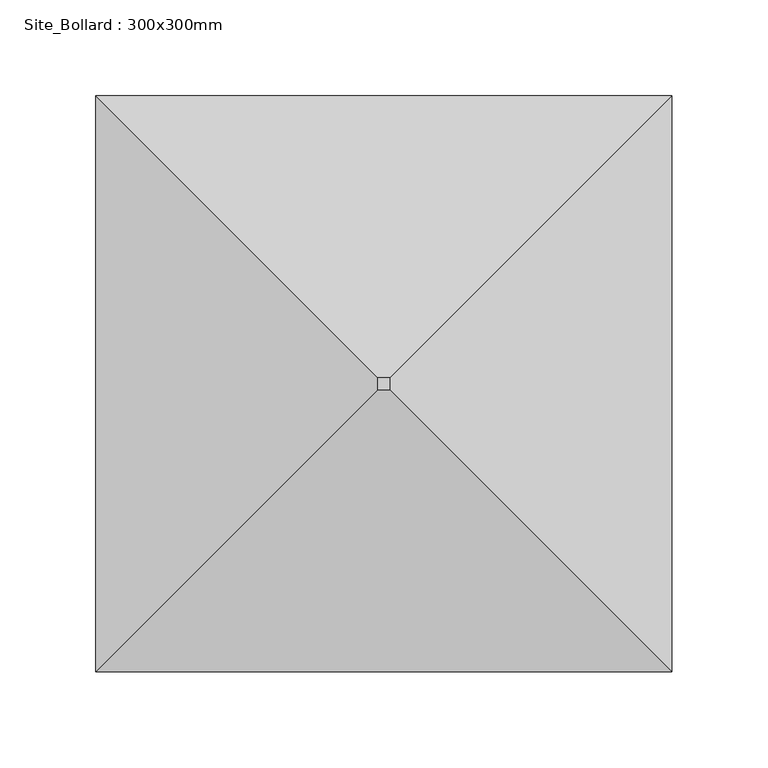
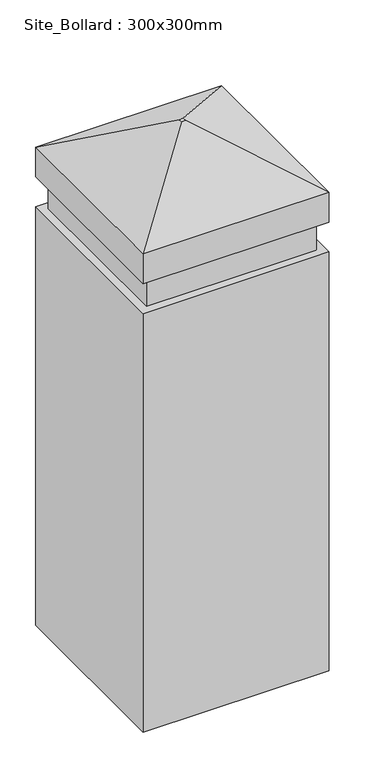
"""IFC4 building model written with IfcOpenShell, lengths in millimetres: geographic element geometry, Site_Bollard : 300x300mm."""

import ifcopenshell
import ifcopenshell.guid

model = None  # the IFC model being written
_history = None  # IfcOwnerHistory: only IFC2X3 demands one
_inside = {}  # id of a spatial element -> (the spatial element, [elements in it])
_under = {}  # id of a project, library or spatial element -> (it, [spatial elements below it])
_declared = {}  # id of a project -> (the project, [libraries it declares])
_typed = {}  # id of a type object -> (the type object, [elements of that type])
_made_of = {}  # id of a material, layer set ... -> (it, [elements and type objects made of it])


def new_model(schema):
    """Start an empty IFC model of exactly this schema.

    Asked for "IFC4X3", IfcOpenShell would pick the latest addendum, in which some entities
    have other attributes; the version numbers below select the first issue.
    IFC2X3 requires an IfcOwnerHistory on every rooted entity: one is made here for all.
    """
    global model, _history
    if schema == "IFC4X3":
        model = ifcopenshell.file(schema_version=(4, 3, 0, 0))
    else:
        model = ifcopenshell.file(schema=schema)
    _inside.clear()
    _under.clear()
    _declared.clear()
    _typed.clear()
    _made_of.clear()
    _history = None
    if model.schema == "IFC2X3":
        org = make("IfcOrganization", Name="unknown")
        user = make(
            "IfcPersonAndOrganization",
            ThePerson=make("IfcPerson", FamilyName="unknown"),
            TheOrganization=org,
        )
        app = make(
            "IfcApplication",
            ApplicationDeveloper=org,
            Version="unknown",
            ApplicationFullName="unknown",
            ApplicationIdentifier="unknown",
        )
        _history = make(
            "IfcOwnerHistory",
            OwningUser=user,
            OwningApplication=app,
            ChangeAction="ADDED",
            CreationDate=0,
        )
    return model


def make(cls, **values):
    """One entity of the class cls with the attributes given. An attribute that is None is left unset."""
    return model.create_entity(
        cls, **{name: value for name, value in values.items() if value is not None}
    )


def rooted(cls, **values):
    """An entity with a GlobalId (a new one), such as an element, a storey or a relation."""
    return make(cls, GlobalId=ifcopenshell.guid.new(), OwnerHistory=_history, **values)


def si_unit(unit_type, name, prefix=None):
    """IfcSIUnit, for example si_unit("LENGTHUNIT", "METRE", prefix="MILLI")."""
    return make("IfcSIUnit", UnitType=unit_type, Prefix=prefix, Name=name)


def assignment(units):
    """IfcUnitAssignment: the units of a project."""
    return None if units is None else make("IfcUnitAssignment", Units=units)


def point(xyz):
    """IfcCartesianPoint."""
    return None if xyz is None else make("IfcCartesianPoint", Coordinates=xyz)


def direction(xyz):
    """IfcDirection."""
    return None if xyz is None else make("IfcDirection", DirectionRatios=xyz)


def frame(location, z_axis=None, x_axis=None):
    """IfcAxis2Placement3D, a coordinate frame: its origin and axes. An axis left out is left unset."""
    return make(
        "IfcAxis2Placement3D",
        Location=point(location),
        Axis=direction(z_axis),
        RefDirection=direction(x_axis),
    )


def origin():
    """The frame at (0, 0, 0) with its axes left unset."""
    return frame((0.0, 0.0, 0.0))


def origin_with_axes():
    """The frame at (0, 0, 0) with the z axis (0, 0, 1) and the x axis (1, 0, 0) written out."""
    return frame((0.0, 0.0, 0.0), z_axis=(0.0, 0.0, 1.0), x_axis=(1.0, 0.0, 0.0))


def place(relative_to, where):
    """IfcLocalPlacement: puts the frame where relative to a parent placement (None: the world)."""
    return make(
        "IfcLocalPlacement", PlacementRelTo=relative_to, RelativePlacement=where
    )


def context(
    kind, dimensions, precision=None, world=None, true_north=None, identifier=None
):
    """IfcGeometricRepresentationContext, for example the 3D "Model" context."""
    return make(
        "IfcGeometricRepresentationContext",
        ContextIdentifier=identifier,
        ContextType=kind,
        CoordinateSpaceDimension=dimensions,
        Precision=precision,
        WorldCoordinateSystem=world,
        TrueNorth=true_north,
    )


def project(units=None, contexts=None):
    """IfcProject with its units and contexts."""
    return rooted(
        "IfcProject",
        Name="project",
        RepresentationContexts=contexts,
        UnitsInContext=assignment(units),
    )


def spatial(cls, under=None, at=None, **own):
    """A site, building, storey or space (cls), placed at a placement, below another one or the project."""
    s = rooted(cls, ObjectPlacement=at, **own)
    if under is not None:
        _under.setdefault(under.id(), (under, []))[1].append(s)
    return s


def polyline(points):
    """IfcPolyline through the points."""
    return make("IfcPolyline", Points=[point(p) for p in points])


def outline(outer, holes=None, kind="AREA"):
    """IfcArbitraryClosedProfileDef: a profile drawn as a closed curve; with holes, ...WithVoids."""
    if holes is None:
        return make("IfcArbitraryClosedProfileDef", ProfileType=kind, OuterCurve=outer)
    return make(
        "IfcArbitraryProfileDefWithVoids",
        ProfileType=kind,
        OuterCurve=outer,
        InnerCurves=holes,
    )


def extrude(swept, where, along, depth):
    """IfcExtrudedAreaSolid: the profile swept, set in the frame where, extruded along a direction by depth."""
    return make(
        "IfcExtrudedAreaSolid",
        SweptArea=swept,
        Position=where,
        ExtrudedDirection=direction(along),
        Depth=depth,
    )


def faces_of(points, faces, orient=None, outer=None):
    """IfcFace entities. A face is a list of loops; a loop is a list of indices into points, from 0.

    orient and outer hold one flag for each loop. By default every Orientation is true, the
    first loop of a face is its IfcFaceOuterBound and the others are IfcFaceBound.
    """
    made = []
    for i, loops in enumerate(faces):
        bounds = []
        for j, loop in enumerate(loops):
            is_outer = j == 0 if outer is None else outer[i][j]
            bounds.append(
                make(
                    "IfcFaceOuterBound" if is_outer else "IfcFaceBound",
                    Bound=make("IfcPolyLoop", Polygon=[points[k] for k in loop]),
                    Orientation=True if orient is None else orient[i][j],
                )
            )
        made.append(make("IfcFace", Bounds=bounds))
    return made


def faceted_brep(points, faces, orient=None, outer=None, voids=None):
    """IfcFacetedBrep: a solid bounded by flat faces; with voids (closed shells), ...WithVoids."""
    shared = [point(p) for p in points]
    hull = make("IfcClosedShell", CfsFaces=faces_of(shared, faces, orient, outer))
    if voids is None:
        return make("IfcFacetedBrep", Outer=hull)
    return make(
        "IfcFacetedBrepWithVoids",
        Outer=hull,
        Voids=[
            make(cls, CfsFaces=faces_of(shared, fs, o, b)) for cls, fs, o, b in voids
        ],
    )


def shape(context_of_items, identifier, shape_type, items):
    """IfcShapeRepresentation: the items that make up one representation, for example the "Body"."""
    return make(
        "IfcShapeRepresentation",
        ContextOfItems=context_of_items,
        RepresentationIdentifier=identifier,
        RepresentationType=shape_type,
        Items=items,
    )


def source(mapping_origin, context_of_items, identifier, shape_type, items):
    """IfcRepresentationMap: a shape defined once, which mapped items show again and again."""
    return make(
        "IfcRepresentationMap",
        MappingOrigin=mapping_origin,
        MappedRepresentation=shape(context_of_items, identifier, shape_type, items),
    )


def transform(
    local_origin,
    x_axis=None,
    y_axis=None,
    z_axis=None,
    scale=None,
    scale2=None,
    scale3=None,
    uniform=True,
):
    """IfcCartesianTransformationOperator3D, or its non-uniform kind. x_axis, y_axis, z_axis: its Axis1, 2, 3."""
    if uniform:
        return make(
            "IfcCartesianTransformationOperator3D",
            Axis1=direction(x_axis),
            Axis2=direction(y_axis),
            LocalOrigin=point(local_origin),
            Scale=scale,
            Axis3=direction(z_axis),
        )
    return make(
        "IfcCartesianTransformationOperator3DnonUniform",
        Axis1=direction(x_axis),
        Axis2=direction(y_axis),
        LocalOrigin=point(local_origin),
        Scale=scale,
        Axis3=direction(z_axis),
        Scale2=scale2,
        Scale3=scale3,
    )


def mapped(mapping_source, mapping_target):
    """IfcMappedItem: shows the shape of a source again, moved by a transform."""
    return make(
        "IfcMappedItem", MappingSource=mapping_source, MappingTarget=mapping_target
    )


def made_of(thing, what):
    """Note that an element or type object is made of a material, layer set ...; save() writes the relation."""
    if what is not None:
        _made_of.setdefault(what.id(), (what, []))[1].append(thing)
    return thing


def element(
    cls,
    number,
    at=None,
    inside=None,
    cuts=None,
    type_object=None,
    material=None,
    context=None,
    identifier="Body",
    shape_type=None,
    held_by="IfcProductDefinitionShape",
    body=None,
    shapes=None,
    **own,
):
    """One element of the class cls, such as IfcWall. Its Tag is "e" and its number.

    at: its placement. inside: the storey or other place that contains it. cuts: it is an
    opening in that element (IfcRelVoidsElement). A single representation is given by context,
    identifier, shape_type and body (its items); several are given by shapes. held_by: the class
    of the entity that holds the representations. save() writes the other relations.
    """
    e = rooted(cls, Tag="e%d" % number, ObjectPlacement=at, **own)
    if body is not None:
        shapes = [shape(context, identifier, shape_type, body)]
    if shapes is not None:
        e.Representation = make(held_by, Representations=shapes)
    if inside is not None:
        _inside.setdefault(inside.id(), (inside, []))[1].append(e)
    if cuts is not None:
        rooted(
            "IfcRelVoidsElement", RelatingBuildingElement=cuts, RelatedOpeningElement=e
        )
    if type_object is not None:
        _typed.setdefault(type_object.id(), (type_object, []))[1].append(e)
    return made_of(e, material)


def aggregate(whole, parts):
    """IfcRelAggregates: a whole, such as a stair, and the parts it consists of."""
    return rooted("IfcRelAggregates", RelatingObject=whole, RelatedObjects=parts)


def save(model, path):
    """Write the relations noted so far, then the file.

    IfcRelAggregates (storeys below a building ...), IfcRelContainedInSpatialStructure (elements
    in a storey), IfcRelDefinesByType, IfcRelAssociatesMaterial and IfcRelDeclares: one each for
    every whole, place, type object, material and project.
    """
    for whole, parts in _under.values():
        aggregate(whole, parts)
    for where, things in _inside.values():
        rooted(
            "IfcRelContainedInSpatialStructure",
            RelatedElements=things,
            RelatingStructure=where,
        )
    for kind, things in _typed.values():
        rooted("IfcRelDefinesByType", RelatedObjects=things, RelatingType=kind)
    for what, things in _made_of.values():
        rooted("IfcRelAssociatesMaterial", RelatedObjects=things, RelatingMaterial=what)
    for by, libraries in _declared.values():
        rooted("IfcRelDeclares", RelatingContext=by, RelatedDefinitions=libraries)
    model.write(path)


def site_bollard_300x300mm_9e5afc0f(model_context):
    return source(origin(), model_context, "Body", "SolidModel", [
        faceted_brep([(5.575, 5.575, 900.0), (-0.775, 5.575, 900.0), (-0.775, -0.775, 900.0), (5.575, -0.775, 900.0), (152.4, 152.4, 815.18125), (152.4, -147.6, 815.18125), (-147.6, -147.6, 815.18125), (-147.6, 152.4, 815.18125)], [[[0, 1, 2, 3]], [[4, 5, 6, 7]], [[4, 7, 1, 0]], [[7, 6, 2, 1]], [[6, 5, 3, 2]], [[5, 4, 0, 3]]]),
        extrude(outline(polyline([(152.4, 152.4), (152.4, -147.6), (-147.6, -147.6), (-147.6, 152.4), (152.4, 152.4)])), frame((0.0, 0.0, 764.38125), z_axis=(0.0, 0.0, 1.0), x_axis=(1.0, 0.0, 0.0)), (0.0, 0.0, 1.0), 50.8),
        extrude(outline(polyline([(139.7, 139.7), (139.7, -134.9), (-134.9, -134.9), (-134.9, 139.7), (139.7, 139.7)])), frame((0.0, 0.0, 713.58125), z_axis=(0.0, 0.0, 1.0), x_axis=(1.0, 0.0, 0.0)), (0.0, 0.0, 1.0), 50.8),
        extrude(outline(polyline([(152.4, 152.4), (152.4, -147.6), (-147.6, -147.6), (-147.6, 152.4), (152.4, 152.4)])), origin_with_axes(), (0.0, 0.0, 1.0), 713.58125),
    ])


if __name__ == "__main__":
    model = new_model("IFC4")
    model_context = context("Model", 3, world=origin())
    ifc_project = project(units=[si_unit("LENGTHUNIT", "METRE", prefix="MILLI")], contexts=[model_context])
    site = spatial("IfcSite", under=ifc_project)
    building = spatial("IfcBuilding", under=site)
    placement = place(None, origin())
    site_bollard_300x300mm_shape = site_bollard_300x300mm_9e5afc0f(model_context)
    element("IfcGeographicElement", 1, ObjectType="Site_Bollard : 300x300mm", at=placement, inside=building, context=model_context, shape_type="MappedRepresentation", body=[
        mapped(site_bollard_300x300mm_shape, transform((0.0, 0.0, 0.0), x_axis=(1.0, 0.0, 0.0), y_axis=(0.0, 1.0, 0.0), z_axis=(0.0, 0.0, 1.0))),
    ])
    save(model, "model.ifc")

# Revit data of these elements
# Project information
#   Project Status = "Project Status"
#   Client Name = "Revit Project"
#   Project Address = "LIMERICK INSTITUTE of TECHNOLOGY"
#   Project Name = "Commercial Units"
#   Project Number = "01"
# Type "Site_Bollard : 300x300mm"
#   Material = Concrete - Precast Concrete
# Element 1 (IfcGeographicElement, "Site_Bollard : 300x300mm")
#   Materials on its faces: "Concrete - Precast Concrete"
# Materials
#   "Concrete - Precast Concrete": class "Concrete", colour RGB 198 187 187, transparency 0
